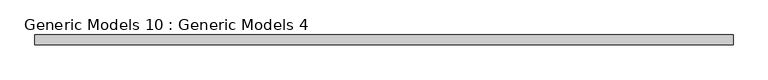
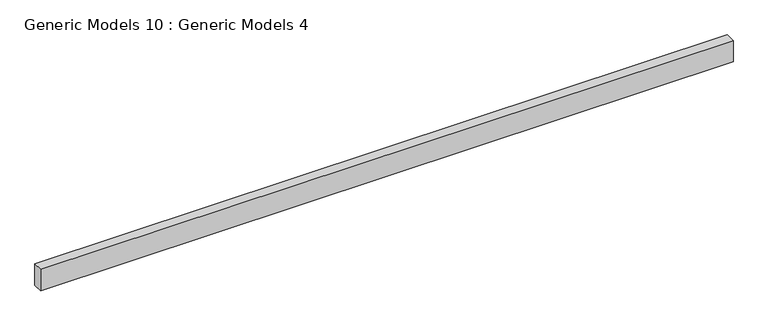
"""IFC4 building model written with IfcOpenShell, lengths in millimetres: proxy geometry, Generic Models 10 : Generic Models 4."""

from ifc_helpers import new_model, si_unit, frame, origin, place, context, project, spatial, polyline, outline, extrude, source, transform, mapped, element, save


def generic_models_10_generic_models_4_a0983e47(model_context):
    return source(origin(), model_context, "Body", "SweptSolid", [
        extrude(outline(polyline([(2196.9263704, -5467.4125551), (2196.9263704, -5645.2125551), (-10256.7421316, -5645.2125551), (-10256.7421316, -5467.4125551), (2196.9263704, -5467.4125551)])), frame((0.0, 0.0, 126393.2620697), z_axis=(0.0, 0.0, 1.0), x_axis=(1.0, 0.0, 0.0)), (0.0, 0.0, 1.0), 406.4),
    ])


if __name__ == "__main__":
    model = new_model("IFC4")
    model_context = context("Model", 3, world=origin())
    ifc_project = project(units=[si_unit("LENGTHUNIT", "METRE", prefix="MILLI")], contexts=[model_context])
    site = spatial("IfcSite", under=ifc_project)
    building = spatial("IfcBuilding", under=site)
    placement = place(None, origin())
    generic_models_10_generic_models_4_shape = generic_models_10_generic_models_4_a0983e47(model_context)
    element("IfcBuildingElementProxy", 1, Name="Generic Models 10 : Generic Models 4", ObjectType="Generic Models 10 : Generic Models 4", at=placement, inside=building, context=model_context, shape_type="MappedRepresentation", body=[
        mapped(generic_models_10_generic_models_4_shape, transform((0.0, 0.0, 0.0), x_axis=(1.0, 0.0, 0.0), y_axis=(0.0, 1.0, 0.0), z_axis=(0.0, 0.0, 1.0))),
    ])
    save(model, "model.ifc")

# Revit data of these elements
# Element 1 (IfcBuildingElementProxy, "Generic Models 10 : Generic Models 4")
#   Materials on its faces: "_STRUCTURAL MEMBER (SEE STRUCT. DWGS)"
# Materials
#   "_STRUCTURAL MEMBER (SEE STRUCT. DWGS)": class "Generic", colour RGB 209 182 141, transparency 0, Cost = 0
